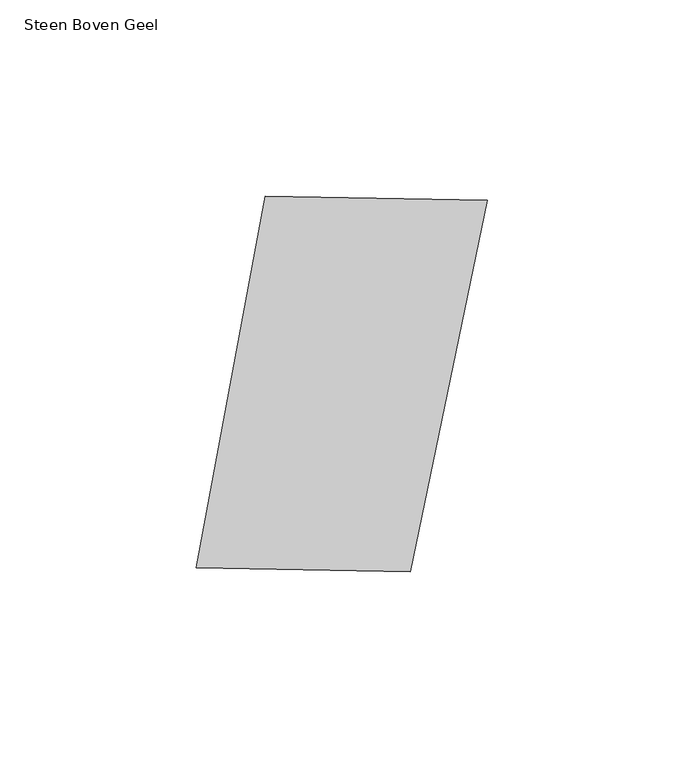
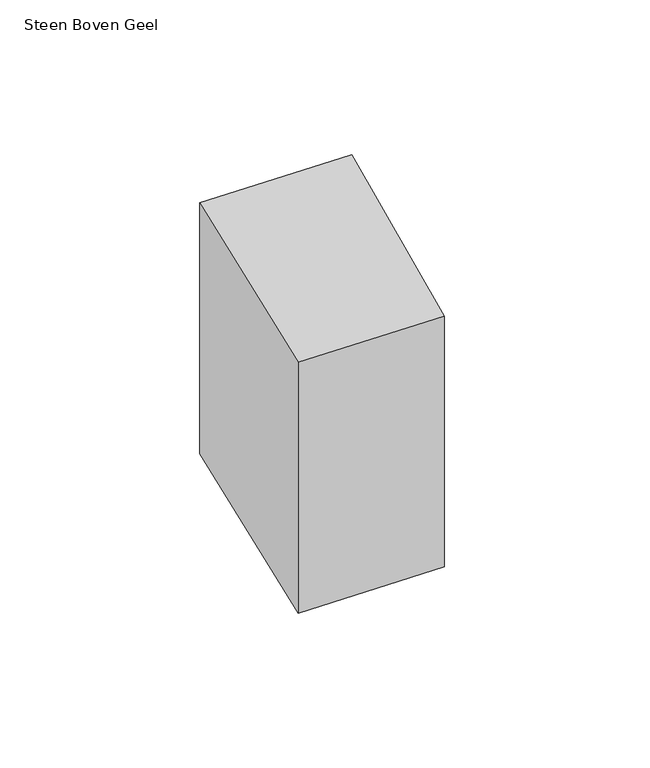
"""IFC4 building model written with IfcOpenShell, lengths in millimetres: proxy geometry, 00_GMA_steen_versie_4 : Steen Boven Geel."""

from ifc_helpers import new_model, si_unit, origin, origin_with_axes, place, context, project, spatial, polyline, outline, extrude, source, transform, mapped, element, save


def steen_boven_geel_fad343a9(model_context):
    return source(origin(), model_context, "Body", "SweptSolid", [
        extrude(outline(polyline([(110.927945, 118.5048593), (91.1994464, 23.7704113), (36.6587194, 24.8022214), (54.2711054, 119.5601524), (110.927945, 118.5048593)])), origin_with_axes(), (0.0, 0.0, 1.0), 100.0),
    ])


if __name__ == "__main__":
    model = new_model("IFC4")
    model_context = context("Model", 3, world=origin())
    ifc_project = project(units=[si_unit("LENGTHUNIT", "METRE", prefix="MILLI")], contexts=[model_context])
    site = spatial("IfcSite", under=ifc_project)
    building = spatial("IfcBuilding", under=site)
    placement = place(None, origin())
    steen_boven_geel_shape = steen_boven_geel_fad343a9(model_context)
    element("IfcBuildingElementProxy", 1, Name="00_GMA_steen_versie_4 : Steen Boven Geel", ObjectType="00_GMA_steen_versie_4 : Steen Boven Geel", at=placement, inside=building, context=model_context, shape_type="MappedRepresentation", body=[
        mapped(steen_boven_geel_shape, transform((0.0, 0.0, 0.0), x_axis=(1.0, 0.0, 0.0), y_axis=(0.0, 1.0, 0.0), z_axis=(0.0, 0.0, 1.0))),
    ])
    save(model, "model.ifc")

# Revit data of these elements
# Type "00_GMA_steen_versie_4 : Steen Boven Geel"
#   StootVoegHalfBoven [instance default] = 5 mm
#   StootVoegHalf [instance default] = 5 mm
#   StootVoegBreedteOnder = 10 mm
#   StootVoegBreedteBoven = 10 mm
#   Steendikte = 100 mm
#   LintVoegOnderHalf = 5 mm
#   LintVoegOnder = 10 mm
#   LintVoegBovenHalf = 0 mm
#   LintVoegBoven = 0 mm
#   materiaal = 21_steen_geel
#   MateriaalVoeg = none
#   Default Elevation = 0
# Element 1 (IfcBuildingElementProxy, "00_GMA_steen_versie_4 : Steen Boven Geel")
#   Materials on its faces: "21_steen_geel"
# Materials
#   "21_steen_geel": class "Unassigned", colour RGB 202 202 0, transparency 0, Cost = 0
